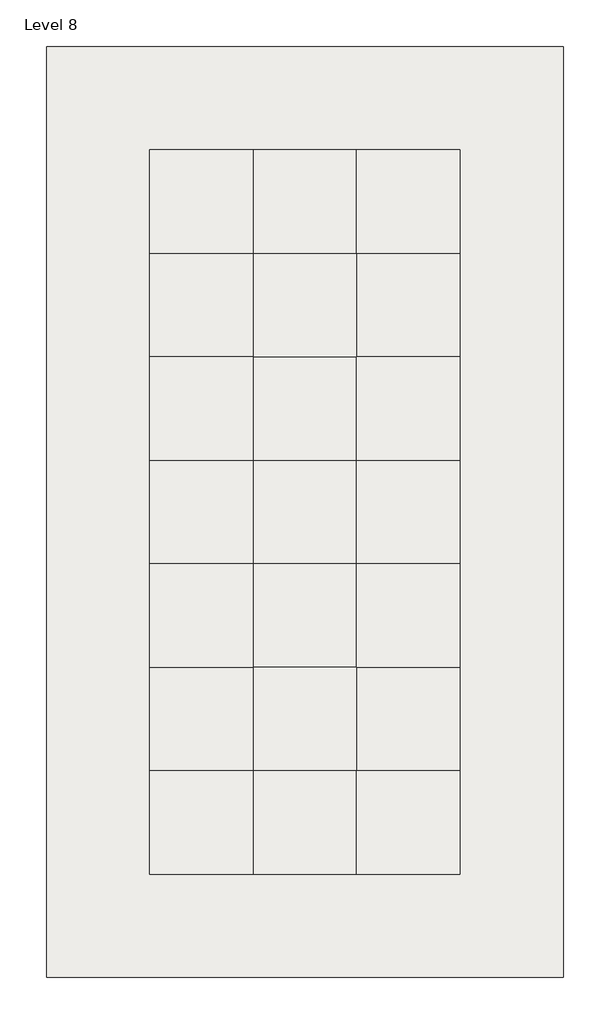
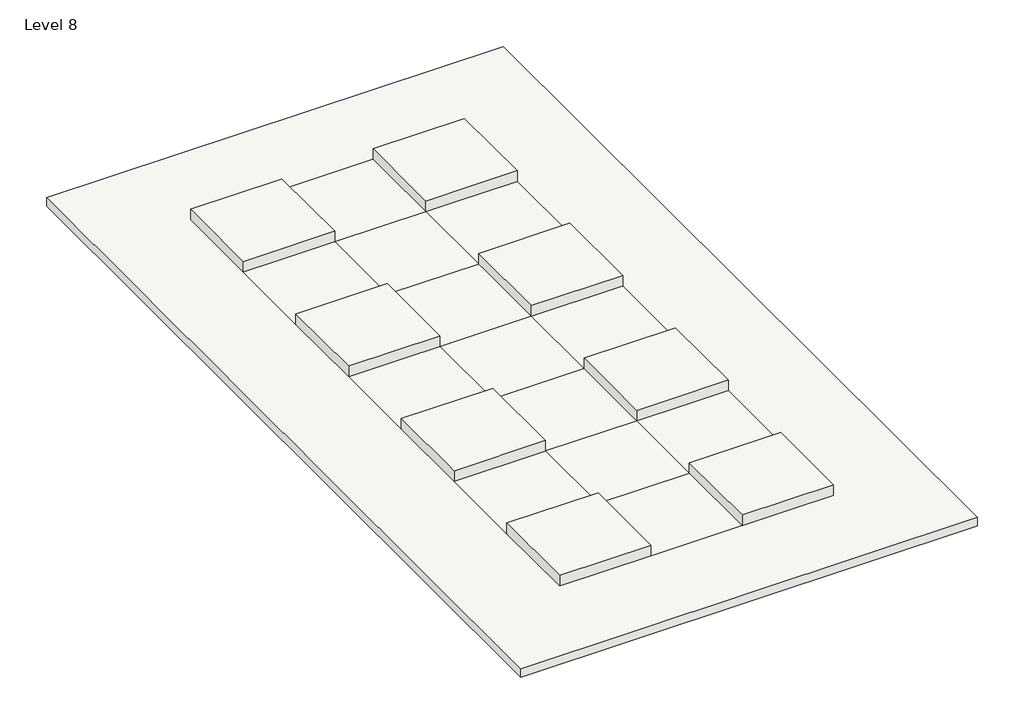
# One storey: 9 roofs.
# Revit data of these elements (continued)
# Materials (continued)
#   "Bauder_ProtectionMat_BauderGREEN-FSM-600": class "Unassigned", colour RGB 255 255 255, transparency 0, Mtrl_Author = "AM", Mtrl_AuthorizedBy = "bimstore", Mtrl_DistributedBy = "www.bimstore.co", Mtrl_AccessibilityPerformance = "n/a", Mtrl_AssetIdentifier = "Please record on commissioning", Mtrl_AssetType = "Fixed", Mtrl_BarCode = "Please record on commissioning", Mtrl_ClassificationName = "Uniclass2017", Mtrl_ClassificationValue = "Pr_20_96_71_64", Mtrl_CodePerformance = "n/a", Mtrl_Color = "n/a", Mtrl_Constituents = "n/a", Mtrl_CreatedBy = "technical@bauder.co.uk", Mtrl_CreatedOn = "2023-02-10 T00:00:00", Mtrl_DocumentationCertificates = "https://www.bimstore.co/products/extensive-green-roof-system-wildflower-blanket/document/product-certificates", Mtrl_DocumentationInstallationGuide = "https://www.bimstore.co/products/extensive-green-roof-system-wildflower-blanket/document/installation-guide", Mtrl_DocumentationLiterature = "https://www.bimstore.co/products/extensive-green-roof-system-wildflower-blanket/document/product-literature", Mtrl_DocumentationMaintenance = "https://www.bimstore.co/products/extensive-green-roof-system-wildflower-blanket/document/maintenance-information", Mtrl_DocumentationTechnical = "https://www.bimstore.co/products/extensive-green-roof-system-wildflower-blanket/document/technical-data-sheet", Mtrl_DurationUnit = "Year", Mtrl_Features = "n/a", Mtrl_Finish = "n/a", Mtrl_Grade = "n/a", Mtrl_InstallationDate = "Please record on commissioning", Mtrl_ManufacturerName = "Bauder Ltd", Mtrl_Material = "Polyester and Polypropylene Fibre", Mtrl_ModelNumber = "BauderGREEN-FSM-600", Mtrl_ModelReference = "Protection Mat", Mtrl_ProductionYear = "2023", Mtrl_ReferencedStandard = "n/a", Mtrl_Shape = "n/a", Mtrl_Size = "n/a", Mtrl_SpareParts = "n/a", Mtrl_TypeName = "BauderGREEN-FSM-600", Mtrl_WarrantyDescription = "As part of Bauder system guarantee, per specification", Mtrl_WarrantyDurationUnit = "Year", Mtrl_WarrantyGuarantorLabor = "technical@bauder.co.uk", Mtrl_WarrantyGuarantorParts = "technical@bauder.co.uk", Mtrl_WarrantyStartDate = "Please record on commissioning", Mtrl_IfcExportAs = "IfcRoofType", Mtrl_IfcExportType = "FLAT_ROOF", Mtrl_BIMObjectName = "Bauder_ProtectionMat_BauderGREEN-FSM-600", Mtrl_NBSDescription = "n/a", Mtrl_NBSNote = "n/a", Mtrl_NBSObjectName = "n/a", Mtrl_NBSOfficeMasterTag = "n/a", Mtrl_NBSReference = "Q37", Mtrl_Ballast = "n/a", Mtrl_CarrierMembraneAttachment = "n/a", Mtrl_CarrierMembraneFixing = "n/a", Mtrl_CarrierMembraneType = "n/a", Mtrl_Certification = "Comply with GRO Green Roof Code of Practice and FLL Standards", Mtrl_DetailWorkAncillaryItems = "Detail as per project specific Bauder Specification", Mtrl_DetailWorkCoverStrips = "Detail as per project specific Bauder Specification", Mtrl_DetailWorkFlashings = "Detail as per project specific Bauder Specification", Mtrl_DetailWorkSkirtingsAndUpstands = "Detail as per project specific Bauder Specification", Mtrl_DetailWorkWeltedDrips = "Detail as per project specific Bauder Specification", Mtrl_EdgeRestraints = "Detail as per project specific Bauder Specification", Mtrl_FillToPerimeterUpstands = "n/a", Mtrl_FilterLayer = "n/a", Mtrl_InsulationAttachment = "As per project specific Bauder Specification", Mtrl_InsulationFixing = "As per project specific Bauder Specification", Mtrl_InsulationType = "As per project specific Bauder Specification", Mtrl_IsolatingLayer = "n/a", Mtrl_LiquidAppliedWaterproofCoatingReinforcement = "As per project specific Bauder Specification", Mtrl_LiquidAppliedWaterproofCoatingSurfaceTreatment = "As per project specific Bauder Specification", Mtrl_LiquidAppliedWaterproofCoatingType = "As per project specific Bauder Specification", Mtrl_LiquidAppliedWaterproofCoatingWearingCourse = "As per project specific Bauder Specification", Mtrl_LowerProtectionLayer = "n/a", Mtrl_MoistureControlDrainageAncillaries = "n/a", Mtrl_MoistureControlDrainageLayer = "n/a", Mtrl_MoistureControlFilterMembrane = "n/a", Mtrl_MoistureControlMoistureRetentionMat = "n/a", Mtrl_OverlayFixing = "n/a", Mtrl_OverlayType = "n/a", Mtrl_PlantingSystemsAntierosionMat = "n/a", Mtrl_PlantingSystemsPlantingMedium = "As per project specific Bauder Specification", Mtrl_PlantingSystemsVegetation = "As per project specific Bauder Specification", Mtrl_PlantingSystemsVegetationBarrier = "As per project specific Bauder Specification", Mtrl_PreparationExistingSubstrates = "n/a", Mtrl_PreparationHorizontalWork = "n/a", Mtrl_PreparationSkirtingsAndVerticalWork = "n/a", Mtrl_ProjectSpecificationAndDesign = "This BIM Object must be supported by a project specific specification from Bauder, incorporating system build-up, detail design and performance calculations if a full Bauder system warranty is required. Please contact your local Bauder Representative or technical@bauder.co.uk", Mtrl_ProtectionLayer = "n/a", Mtrl_ProtectionProtectionLayer = "n/a", Mtrl_ProtectionRootBarrier = "As per project specific Bauder Specification", Mtrl_ProtectionSeparationLayer = "n/a", Mtrl_SeparatingLayer = "n/a", Mtrl_SurfaceProtection = "n/a", Mtrl_SystemAccessories = "n/a", Mtrl_SystemManufacturer = "Bauder Ltd", Mtrl_Update = "1900-12-31 T23:59:59", Mtrl_UpperProtectionLayer = "n/a", Mtrl_VapourControlLayerAttachment = "As per project specific Bauder Specification", Mtrl_VapourControlLayerAttachment_Bauder = "As per project specific Bauder Specification", Mtrl_VapourControlLayerType = "As per project specific Bauder Specification", Mtrl_WarrantyConsiderations = "All guarantees available for this system are subject to the works being carried out in accordance with the Bauder specification and being installed by a Bauder Approved installer. For full details and further information regarding guarantees and alternative systems please contact your local Bauder Representative or technical@bauder.co.uk", Mtrl_WaterproofCoveringAccessories = "As per project specific Bauder Specification", Mtrl_WaterproofCoveringAttachment = "As per project specific Bauder Specification", Mtrl_WaterproofCoveringFirstLayerAttachment = "As per project specific Bauder Specification", Mtrl_WaterproofCoveringFirstLayerType = "As per project specific Bauder Specification", Mtrl_WaterproofCoveringIntermediateLayerAttachment = "As per project specific Bauder Specification", Mtrl_WaterproofCoveringIntermediateLayerType = "As per project specific Bauder Specification", Mtrl_WaterproofCoveringJoints = "As per project specific Bauder Specification", Mtrl_WaterproofCoveringTopLayerAttachment = "As per project specific Bauder Specification", Mtrl_WaterproofCoveringTopLayerType = "As per project specific Bauder Specification", Mtrl_WaterproofCoveringType = "As per project specific Bauder Specification", Cost = 0, Mtrl_ReplacementCost = 0, Mtrl_NominalDepth = 4 mm, Mtrl_NominalHeight = 0 mm, Mtrl_NominalLength = 0 mm, Mtrl_BimSpecGuid = 0, Mtrl_BSBibleVersion = 17, Mtrl_CurrentRevision = 2, Mtrl_ExpectedLife = 0, Mtrl_SerialNumber = 0, Mtrl_WarrantyDurationLabor = 0, Mtrl_WarrantyDurationParts = 0
#   "Concrete": class "Concrete", colour RGB 120 120 120, transparency 0, Description = "Portland Cement Concrete", Cost = 0
